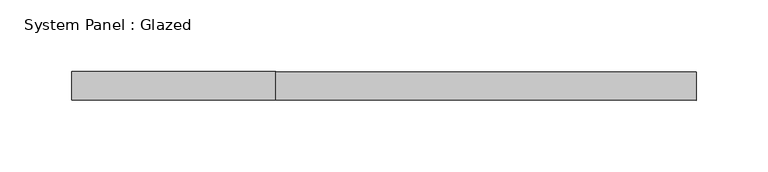
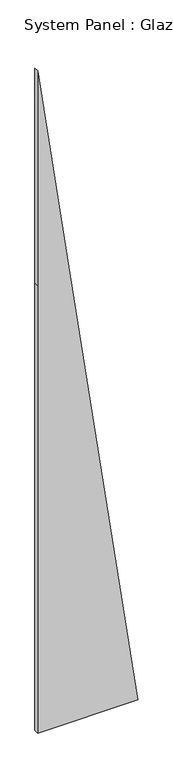
"""IFC4 building model written with IfcOpenShell, lengths in millimetres: plate geometry, System Panel : Glazed."""

from ifc_helpers import new_model, si_unit, frame, origin, place, context, project, spatial, polyline, outline, extrude, source, transform, mapped, element, save


def system_panel_glazed_4e7661e6(model_context):
    return source(origin(), model_context, "Body", "SweptSolid", [
        extrude(outline(polyline([(0.0, -218.4530145), (0.0, 218.4530145), (2052.9059592, -75.7916096), (3048.2357782, -218.4530145), (2060.0, -218.4530145), (0.0, -218.4530145)])), frame((0.0, 0.0, 0.0), z_axis=(0.0, 1.0, 0.0), x_axis=(0.0, 0.0, 1.0)), (0.0, 0.0, 1.0), 20.0),
    ])


if __name__ == "__main__":
    model = new_model("IFC4")
    model_context = context("Model", 3, world=origin())
    ifc_project = project(units=[si_unit("LENGTHUNIT", "METRE", prefix="MILLI")], contexts=[model_context])
    site = spatial("IfcSite", under=ifc_project)
    building = spatial("IfcBuilding", under=site)
    placement = place(None, origin())
    system_panel_glazed_shape = system_panel_glazed_4e7661e6(model_context)
    element("IfcPlate", 1, ObjectType="System Panel : Glazed", at=placement, inside=building, context=model_context, shape_type="MappedRepresentation", body=[
        mapped(system_panel_glazed_shape, transform((0.0, 0.0, 0.0), x_axis=(1.0, 0.0, 0.0), y_axis=(0.0, 1.0, 0.0), z_axis=(0.0, 0.0, 1.0))),
    ])
    save(model, "model.ifc")

# Revit data of these elements
# Type "System Panel : Glazed"
#   COBie.Type = no
# Element 1 (IfcPlate, "System Panel : Glazed")
#   Materials on its faces: "Glass"
# Materials
#   "Glass": class "Glass", colour RGB 0 128 192, transparency 0.75, Description = "Soda Lime Glass", Cost = 0
